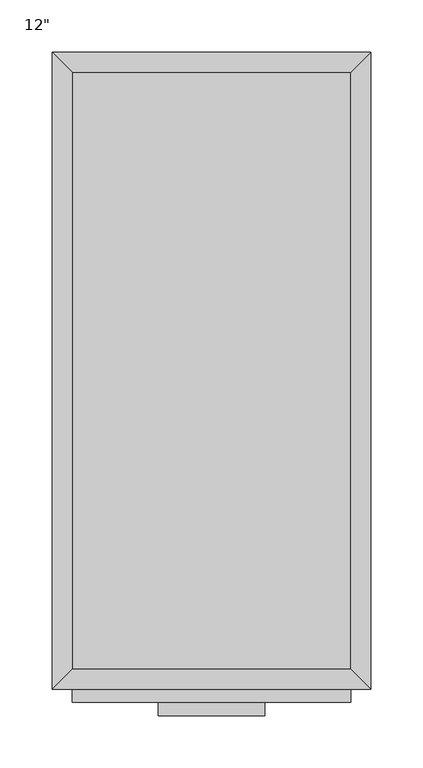
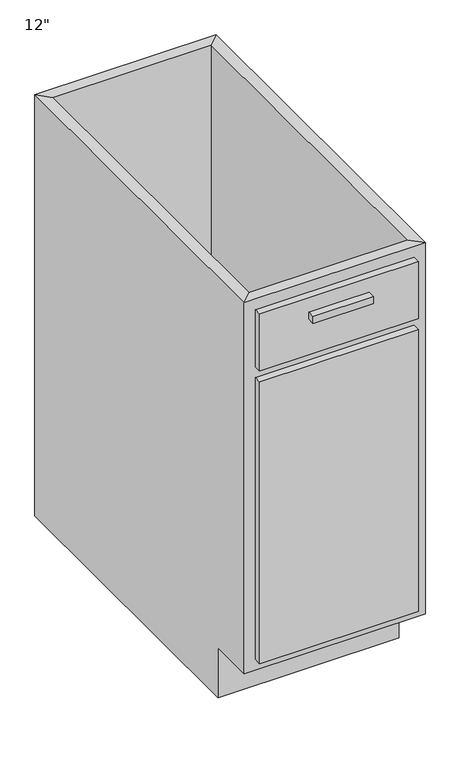
"""IFC4 building model written with IfcOpenShell, lengths in millimetres: furniture geometry."""

from ifc_helpers import new_model, si_unit, frame, origin, place, context, project, spatial, polyline, outline, extrude, faceted_brep, source, transform, mapped, element, save


def furniture_d3494f9b(model_context):
    return source(origin(), model_context, "Body", "SolidModel", [
        faceted_brep([(152.0877049, -590.55, 749.3), (152.0877049, -590.55, 88.9), (-114.6122951, -590.55, 88.9), (-114.6122951, -590.55, 749.3), (-133.6622951, -609.6, 749.3), (171.1377049, -609.6, 749.3), (-133.6622951, -609.6, 88.9), (171.1377049, -609.6, 88.9), (-114.6122951, -533.4, 88.9), (-114.6122951, -19.05, 88.9), (-114.6122951, -19.05, 749.3), (-133.6622951, 0.0, 749.3), (-133.6622951, 0.0, 0.0), (-133.6622951, -533.4, 0.0), (-133.6622951, -533.4, 88.9), (152.0877049, -19.05, 88.9), (152.0877049, -19.05, 749.3), (171.1377049, 0.0, 749.3), (171.1377049, 0.0, 0.0), (152.0877049, -533.4, 88.9), (171.1377049, -533.4, 88.9), (171.1377049, -533.4, 0.0)], [[[0, 1, 2, 3]], [[0, 3, 4, 5]], [[5, 4, 6, 7]], [[2, 1, 7, 6]], [[3, 2, 8, 9, 10]], [[4, 3, 10, 11]], [[6, 4, 11, 12, 13, 14]], [[2, 6, 14, 8]], [[10, 9, 15, 16]], [[11, 10, 16, 17]], [[12, 11, 17, 18]], [[1, 0, 16, 15, 19]], [[0, 5, 17, 16]], [[5, 7, 20, 21, 18, 17]], [[7, 1, 19, 20]], [[8, 19, 15, 9]], [[18, 21, 13, 12]], [[13, 21, 20, 19, 8, 14]]]),
        extrude(outline(polyline([(152.0877049, -19.05), (152.0877049, -590.55), (-114.6122951, -590.55), (-114.6122951, -19.05), (152.0877049, -19.05)])), frame((0.0, 0.0, 88.9), z_axis=(0.0, 0.0, 1.0), x_axis=(1.0, 0.0, 0.0)), (0.0, 0.0, 1.0), 19.05),
        extrude(outline(polyline([(152.0877049, -622.3), (-114.6122951, -622.3), (-114.6122951, -609.6), (152.0877049, -609.6), (152.0877049, -622.3)])), frame((0.0, 0.0, 628.65), z_axis=(0.0, 0.0, 1.0), x_axis=(1.0, 0.0, 0.0)), (0.0, 0.0, 1.0), 101.6),
        extrude(outline(polyline([(152.0877049, -622.3), (-114.6122951, -622.3), (-114.6122951, -609.6), (152.0877049, -609.6), (152.0877049, -622.3)])), frame((0.0, 0.0, 107.95), z_axis=(0.0, 0.0, 1.0), x_axis=(1.0, 0.0, 0.0)), (0.0, 0.0, 1.0), 501.65),
        extrude(outline(polyline([(69.5377049, -635.0), (-32.0622951, -635.0), (-32.0622951, -622.3), (69.5377049, -622.3), (69.5377049, -635.0)])), frame((0.0, 0.0, 692.15), z_axis=(0.0, 0.0, 1.0), x_axis=(1.0, 0.0, 0.0)), (0.0, 0.0, 1.0), 12.7),
    ])


if __name__ == "__main__":
    model = new_model("IFC4")
    model_context = context("Model", 3, world=origin())
    ifc_project = project(units=[si_unit("LENGTHUNIT", "METRE", prefix="MILLI")], contexts=[model_context])
    site = spatial("IfcSite", under=ifc_project)
    building = spatial("IfcBuilding", under=site)
    placement = place(None, origin())
    furniture_shape = furniture_d3494f9b(model_context)
    element("IfcFurniture", 1, ObjectType="Vanity Cabinet-Single Door & Drawer : 12\"", at=placement, inside=building, context=model_context, shape_type="MappedRepresentation", body=[
        mapped(furniture_shape, transform((0.0, 0.0, 0.0), x_axis=(1.0, 0.0, 0.0), y_axis=(0.0, 1.0, 0.0), z_axis=(0.0, 0.0, 1.0))),
    ])
    save(model, "model.ifc")

# Revit data of these elements
# Type "Vanity Cabinet-Single Door & Drawer : 12\""
#   Assembly Code = "C1030410"
#   Depth = 2' - 0"
#   Height = 2' - 5 1/2"
#   Toe Depth = 0' - 3"
#   Toe Height = 0' - 3 1/2"
#   Width = 1' - 0"
#   Cabinet Material = none
#   Door/Drawer Material = none
#   Handle Material = Cabinets - Handles
# Element 1 (IfcFurniture, "Vanity Cabinet-Single Door & Drawer : 12\"")
#   Materials on its faces: "Cabinets", "Cabinets - Handles"
# Materials
#   "Cabinets - Handles": class "Metal", colour RGB 57 57 57, transparency 0
#   "Cabinets": class "Miscellaneous", colour RGB 249 249 249, transparency 0
